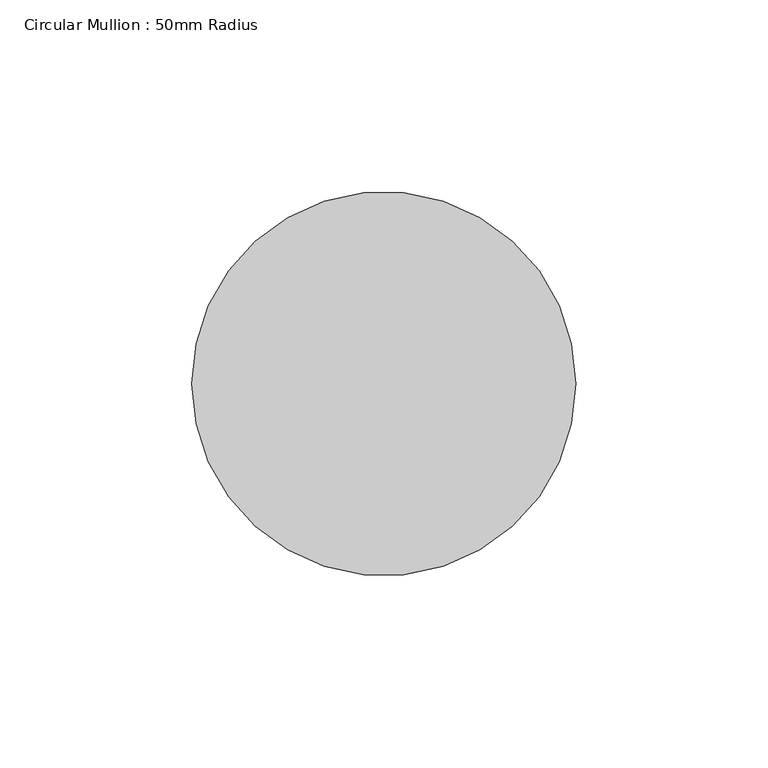
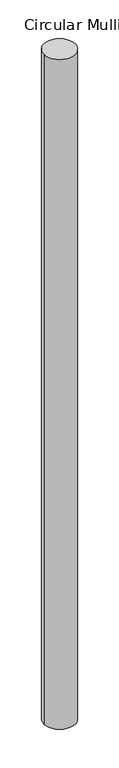
"""IFC4 building model written with IfcOpenShell, lengths in millimetres: member geometry, Circular Mullion : 50mm Radius."""

from ifc_helpers import new_model, si_unit, point, frame, frame_2d, origin, place, context, project, spatial, circle_curve, trimmed, segment, composite_curve, outline, extrude, source, transform, mapped, element, save


def circular_mullion_50mm_radius_27e57362(model_context):
    return source(origin(), model_context, "Body", "SweptSolid", [
        extrude(outline(composite_curve([segment(trimmed(circle_curve(frame_2d((-50.0, 0.0)), 50.0), [point((0.0, 0.0))], [point((-100.0, 0.0))], False, "CARTESIAN"), True, "CONTINUOUS"), segment(trimmed(circle_curve(frame_2d((-50.0, 0.0)), 50.0), [point((-100.0, 0.0))], [point((0.0, 0.0))], False, "CARTESIAN"), True, "CONTINUOUS")], self_intersect=False)), frame((0.0, 0.0, -2246.2835087), z_axis=(0.0, 0.0, 1.0), x_axis=(1.0, 0.0, 0.0)), (0.0, 0.0, 1.0), 2246.2835087),
    ])


if __name__ == "__main__":
    model = new_model("IFC4")
    model_context = context("Model", 3, world=origin())
    ifc_project = project(units=[si_unit("LENGTHUNIT", "METRE", prefix="MILLI")], contexts=[model_context])
    site = spatial("IfcSite", under=ifc_project)
    building = spatial("IfcBuilding", under=site)
    placement = place(None, origin())
    circular_mullion_50mm_radius_shape = circular_mullion_50mm_radius_27e57362(model_context)
    element("IfcMember", 1, ObjectType="Circular Mullion : 50mm Radius", at=placement, inside=building, context=model_context, shape_type="MappedRepresentation", body=[
        mapped(circular_mullion_50mm_radius_shape, transform((0.0, 0.0, 0.0), x_axis=(1.0, 0.0, 0.0), y_axis=(0.0, 1.0, 0.0), z_axis=(0.0, 0.0, 1.0))),
    ])
    save(model, "model.ifc")

# Revit data of these elements
# Type "Circular Mullion : 50mm Radius"
#   built-in parameter 1007350 = 0.164042 (stored number, unit not read)
# Element 1 (IfcMember, "Circular Mullion : 50mm Radius")
#   Materials on its faces: "Aluminium"
# Materials
#   "Aluminium": class "Metal", colour RGB 247 247 247, transparency 0, Description = "Aluminium 6061", Cost = 0
